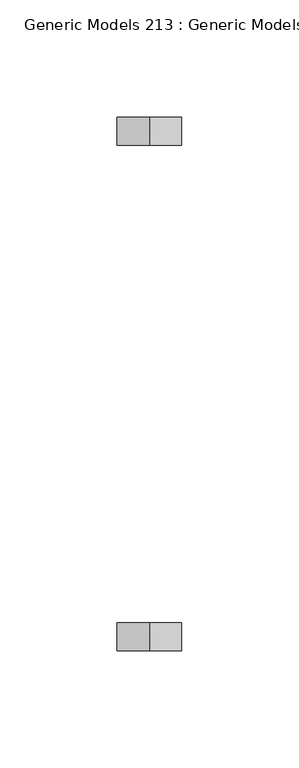
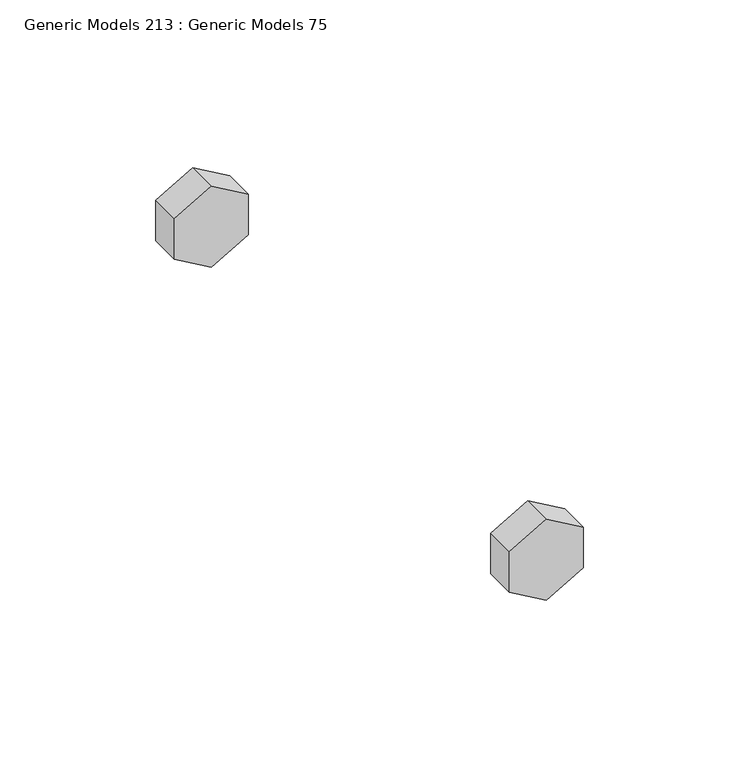
"""IFC4 building model written with IfcOpenShell, lengths in millimetres: proxy geometry, Generic Models 213 : Generic Models 75."""

import ifcopenshell
import ifcopenshell.guid

model = None  # the IFC model being written
_history = None  # IfcOwnerHistory: only IFC2X3 demands one
_inside = {}  # id of a spatial element -> (the spatial element, [elements in it])
_under = {}  # id of a project, library or spatial element -> (it, [spatial elements below it])
_declared = {}  # id of a project -> (the project, [libraries it declares])
_typed = {}  # id of a type object -> (the type object, [elements of that type])
_made_of = {}  # id of a material, layer set ... -> (it, [elements and type objects made of it])


def new_model(schema):
    """Start an empty IFC model of exactly this schema.

    Asked for "IFC4X3", IfcOpenShell would pick the latest addendum, in which some entities
    have other attributes; the version numbers below select the first issue.
    IFC2X3 requires an IfcOwnerHistory on every rooted entity: one is made here for all.
    """
    global model, _history
    if schema == "IFC4X3":
        model = ifcopenshell.file(schema_version=(4, 3, 0, 0))
    else:
        model = ifcopenshell.file(schema=schema)
    _inside.clear()
    _under.clear()
    _declared.clear()
    _typed.clear()
    _made_of.clear()
    _history = None
    if model.schema == "IFC2X3":
        org = make("IfcOrganization", Name="unknown")
        user = make(
            "IfcPersonAndOrganization",
            ThePerson=make("IfcPerson", FamilyName="unknown"),
            TheOrganization=org,
        )
        app = make(
            "IfcApplication",
            ApplicationDeveloper=org,
            Version="unknown",
            ApplicationFullName="unknown",
            ApplicationIdentifier="unknown",
        )
        _history = make(
            "IfcOwnerHistory",
            OwningUser=user,
            OwningApplication=app,
            ChangeAction="ADDED",
            CreationDate=0,
        )
    return model


def make(cls, **values):
    """One entity of the class cls with the attributes given. An attribute that is None is left unset."""
    return model.create_entity(
        cls, **{name: value for name, value in values.items() if value is not None}
    )


def rooted(cls, **values):
    """An entity with a GlobalId (a new one), such as an element, a storey or a relation."""
    return make(cls, GlobalId=ifcopenshell.guid.new(), OwnerHistory=_history, **values)


def si_unit(unit_type, name, prefix=None):
    """IfcSIUnit, for example si_unit("LENGTHUNIT", "METRE", prefix="MILLI")."""
    return make("IfcSIUnit", UnitType=unit_type, Prefix=prefix, Name=name)


def assignment(units):
    """IfcUnitAssignment: the units of a project."""
    return None if units is None else make("IfcUnitAssignment", Units=units)


def point(xyz):
    """IfcCartesianPoint."""
    return None if xyz is None else make("IfcCartesianPoint", Coordinates=xyz)


def direction(xyz):
    """IfcDirection."""
    return None if xyz is None else make("IfcDirection", DirectionRatios=xyz)


def frame(location, z_axis=None, x_axis=None):
    """IfcAxis2Placement3D, a coordinate frame: its origin and axes. An axis left out is left unset."""
    return make(
        "IfcAxis2Placement3D",
        Location=point(location),
        Axis=direction(z_axis),
        RefDirection=direction(x_axis),
    )


def origin():
    """The frame at (0, 0, 0) with its axes left unset."""
    return frame((0.0, 0.0, 0.0))


def place(relative_to, where):
    """IfcLocalPlacement: puts the frame where relative to a parent placement (None: the world)."""
    return make(
        "IfcLocalPlacement", PlacementRelTo=relative_to, RelativePlacement=where
    )


def context(
    kind, dimensions, precision=None, world=None, true_north=None, identifier=None
):
    """IfcGeometricRepresentationContext, for example the 3D "Model" context."""
    return make(
        "IfcGeometricRepresentationContext",
        ContextIdentifier=identifier,
        ContextType=kind,
        CoordinateSpaceDimension=dimensions,
        Precision=precision,
        WorldCoordinateSystem=world,
        TrueNorth=true_north,
    )


def project(units=None, contexts=None):
    """IfcProject with its units and contexts."""
    return rooted(
        "IfcProject",
        Name="project",
        RepresentationContexts=contexts,
        UnitsInContext=assignment(units),
    )


def spatial(cls, under=None, at=None, **own):
    """A site, building, storey or space (cls), placed at a placement, below another one or the project."""
    s = rooted(cls, ObjectPlacement=at, **own)
    if under is not None:
        _under.setdefault(under.id(), (under, []))[1].append(s)
    return s


def polyline(points):
    """IfcPolyline through the points."""
    return make("IfcPolyline", Points=[point(p) for p in points])


def outline(outer, holes=None, kind="AREA"):
    """IfcArbitraryClosedProfileDef: a profile drawn as a closed curve; with holes, ...WithVoids."""
    if holes is None:
        return make("IfcArbitraryClosedProfileDef", ProfileType=kind, OuterCurve=outer)
    return make(
        "IfcArbitraryProfileDefWithVoids",
        ProfileType=kind,
        OuterCurve=outer,
        InnerCurves=holes,
    )


def extrude(swept, where, along, depth):
    """IfcExtrudedAreaSolid: the profile swept, set in the frame where, extruded along a direction by depth."""
    return make(
        "IfcExtrudedAreaSolid",
        SweptArea=swept,
        Position=where,
        ExtrudedDirection=direction(along),
        Depth=depth,
    )


def shape(context_of_items, identifier, shape_type, items):
    """IfcShapeRepresentation: the items that make up one representation, for example the "Body"."""
    return make(
        "IfcShapeRepresentation",
        ContextOfItems=context_of_items,
        RepresentationIdentifier=identifier,
        RepresentationType=shape_type,
        Items=items,
    )


def source(mapping_origin, context_of_items, identifier, shape_type, items):
    """IfcRepresentationMap: a shape defined once, which mapped items show again and again."""
    return make(
        "IfcRepresentationMap",
        MappingOrigin=mapping_origin,
        MappedRepresentation=shape(context_of_items, identifier, shape_type, items),
    )


def transform(
    local_origin,
    x_axis=None,
    y_axis=None,
    z_axis=None,
    scale=None,
    scale2=None,
    scale3=None,
    uniform=True,
):
    """IfcCartesianTransformationOperator3D, or its non-uniform kind. x_axis, y_axis, z_axis: its Axis1, 2, 3."""
    if uniform:
        return make(
            "IfcCartesianTransformationOperator3D",
            Axis1=direction(x_axis),
            Axis2=direction(y_axis),
            LocalOrigin=point(local_origin),
            Scale=scale,
            Axis3=direction(z_axis),
        )
    return make(
        "IfcCartesianTransformationOperator3DnonUniform",
        Axis1=direction(x_axis),
        Axis2=direction(y_axis),
        LocalOrigin=point(local_origin),
        Scale=scale,
        Axis3=direction(z_axis),
        Scale2=scale2,
        Scale3=scale3,
    )


def mapped(mapping_source, mapping_target):
    """IfcMappedItem: shows the shape of a source again, moved by a transform."""
    return make(
        "IfcMappedItem", MappingSource=mapping_source, MappingTarget=mapping_target
    )


def made_of(thing, what):
    """Note that an element or type object is made of a material, layer set ...; save() writes the relation."""
    if what is not None:
        _made_of.setdefault(what.id(), (what, []))[1].append(thing)
    return thing


def element(
    cls,
    number,
    at=None,
    inside=None,
    cuts=None,
    type_object=None,
    material=None,
    context=None,
    identifier="Body",
    shape_type=None,
    held_by="IfcProductDefinitionShape",
    body=None,
    shapes=None,
    **own,
):
    """One element of the class cls, such as IfcWall. Its Tag is "e" and its number.

    at: its placement. inside: the storey or other place that contains it. cuts: it is an
    opening in that element (IfcRelVoidsElement). A single representation is given by context,
    identifier, shape_type and body (its items); several are given by shapes. held_by: the class
    of the entity that holds the representations. save() writes the other relations.
    """
    e = rooted(cls, Tag="e%d" % number, ObjectPlacement=at, **own)
    if body is not None:
        shapes = [shape(context, identifier, shape_type, body)]
    if shapes is not None:
        e.Representation = make(held_by, Representations=shapes)
    if inside is not None:
        _inside.setdefault(inside.id(), (inside, []))[1].append(e)
    if cuts is not None:
        rooted(
            "IfcRelVoidsElement", RelatingBuildingElement=cuts, RelatedOpeningElement=e
        )
    if type_object is not None:
        _typed.setdefault(type_object.id(), (type_object, []))[1].append(e)
    return made_of(e, material)


def aggregate(whole, parts):
    """IfcRelAggregates: a whole, such as a stair, and the parts it consists of."""
    return rooted("IfcRelAggregates", RelatingObject=whole, RelatedObjects=parts)


def save(model, path):
    """Write the relations noted so far, then the file.

    IfcRelAggregates (storeys below a building ...), IfcRelContainedInSpatialStructure (elements
    in a storey), IfcRelDefinesByType, IfcRelAssociatesMaterial and IfcRelDeclares: one each for
    every whole, place, type object, material and project.
    """
    for whole, parts in _under.values():
        aggregate(whole, parts)
    for where, things in _inside.values():
        rooted(
            "IfcRelContainedInSpatialStructure",
            RelatedElements=things,
            RelatingStructure=where,
        )
    for kind, things in _typed.values():
        rooted("IfcRelDefinesByType", RelatedObjects=things, RelatingType=kind)
    for what, things in _made_of.values():
        rooted("IfcRelAssociatesMaterial", RelatedObjects=things, RelatingMaterial=what)
    for by, libraries in _declared.values():
        rooted("IfcRelDeclares", RelatingContext=by, RelatedDefinitions=libraries)
    model.write(path)


def generic_models_213_generic_models_75_9f8ad40d(model_context):
    return source(origin(), model_context, "Body", "SweptSolid", [
        extrude(outline(polyline([(269069.9462802, 31975.9942029), (269054.1097067, 31975.9942029), (269046.19142, 31989.7090778), (269054.1097067, 32003.4239528), (269069.9462802, 32003.4239528), (269077.864567, 31989.7090778), (269069.9462802, 31975.9942029)])), frame((0.0, 30875.9406612, 0.0), z_axis=(0.0, 1.0, 0.0), x_axis=(0.0, 0.0, 1.0)), (0.0, 0.0, 1.0), 11.90625),
        extrude(outline(polyline([(269069.9462802, 31975.9942029), (269054.1097067, 31975.9942029), (269046.19142, 31989.7090778), (269054.1097067, 32003.4239528), (269069.9462802, 32003.4239528), (269077.864567, 31989.7090778), (269069.9462802, 31975.9942029)])), frame((0.0, 30660.8344112, 0.0), z_axis=(0.0, 1.0, 0.0), x_axis=(0.0, 0.0, 1.0)), (0.0, 0.0, 1.0), 11.90625),
    ])


if __name__ == "__main__":
    model = new_model("IFC4")
    model_context = context("Model", 3, world=origin())
    ifc_project = project(units=[si_unit("LENGTHUNIT", "METRE", prefix="MILLI")], contexts=[model_context])
    site = spatial("IfcSite", under=ifc_project)
    building = spatial("IfcBuilding", under=site)
    placement = place(None, origin())
    generic_models_213_generic_models_75_shape = generic_models_213_generic_models_75_9f8ad40d(model_context)
    element("IfcBuildingElementProxy", 1, Name="Generic Models 213 : Generic Models 75", ObjectType="Generic Models 213 : Generic Models 75", at=placement, inside=building, context=model_context, shape_type="MappedRepresentation", body=[
        mapped(generic_models_213_generic_models_75_shape, transform((0.0, 0.0, 0.0), x_axis=(1.0, 0.0, 0.0), y_axis=(0.0, 1.0, 0.0), z_axis=(0.0, 0.0, 1.0))),
    ])
    save(model, "model.ifc")

# Revit data of these elements
# Element 1 (IfcBuildingElementProxy, "Generic Models 213 : Generic Models 75")
#   Materials on its faces: "3/4\" GALV. THRU BOLTS"
# Materials
#   "3/4\" GALV. THRU BOLTS": class "Generic", colour RGB 105 69 171, transparency 0, Cost = 0
